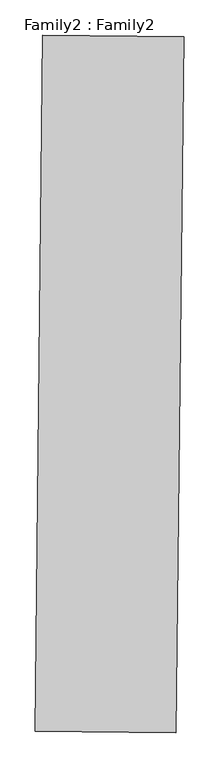
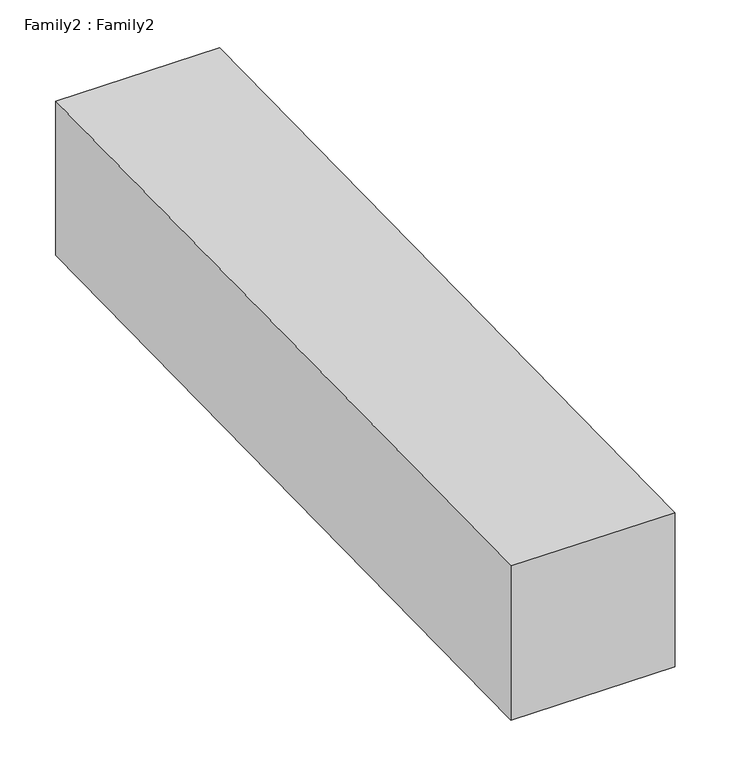
"""IFC4 building model written with IfcOpenShell, lengths in millimetres: proxy geometry, Family2 : Family2."""

from ifc_helpers import new_model, si_unit, origin, place, context, project, spatial, faceted_brep, source, transform, mapped, element, save


def family2_family2_9fa9562e(model_context):
    return source(origin(), model_context, "Body", "Brep", [
        faceted_brep([(-3948.8640696, -6566.8604833, 1.0945136), (-3948.8640696, -6566.8604833, 201.0945136), (-3937.9787249, -5580.7396393, 202.060409), (-3937.9787249, -5580.7396393, 2.060409), (-3748.8728796, -6568.737696, 201.0945136), (-3737.9875349, -5582.6168519, 202.060409), (-3748.8728796, -6568.737696, 1.0945136), (-3737.9875349, -5582.6168519, 2.060409)], [[[0, 1, 2, 3]], [[1, 4, 5, 2]], [[4, 6, 7, 5]], [[6, 0, 3, 7]], [[3, 2, 5, 7]], [[0, 6, 4, 1]]]),
    ])


if __name__ == "__main__":
    model = new_model("IFC4")
    model_context = context("Model", 3, world=origin())
    ifc_project = project(units=[si_unit("LENGTHUNIT", "METRE", prefix="MILLI")], contexts=[model_context])
    site = spatial("IfcSite", under=ifc_project)
    building = spatial("IfcBuilding", under=site)
    placement = place(None, origin())
    family2_family2_shape = family2_family2_9fa9562e(model_context)
    element("IfcBuildingElementProxy", 1, Name="Family2 : Family2", ObjectType="Family2 : Family2", at=placement, inside=building, context=model_context, shape_type="MappedRepresentation", body=[
        mapped(family2_family2_shape, transform((0.0, 0.0, 0.0), x_axis=(1.0, 0.0, 0.0), y_axis=(0.0, 1.0, 0.0), z_axis=(0.0, 0.0, 1.0))),
    ])
    save(model, "model.ifc")

# Revit data of these elements
# Type "Family2 : Family2"
#   Default Elevation = 0
